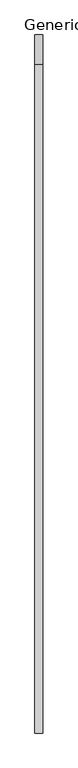
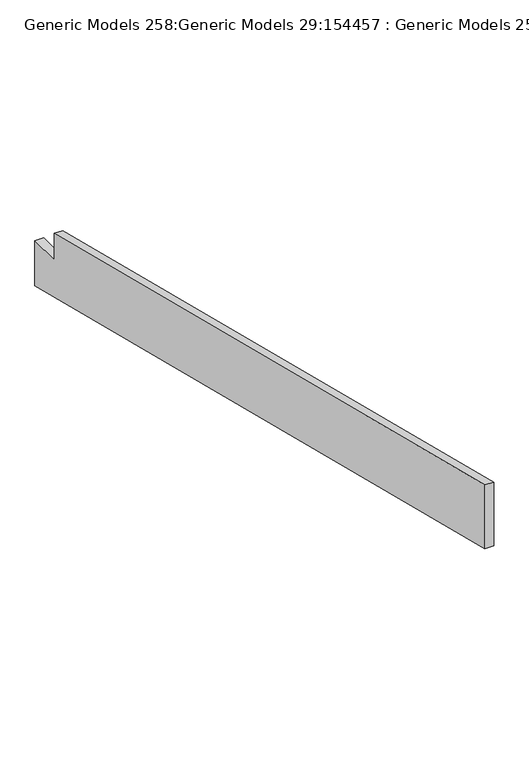
"""IFC4 building model written with IfcOpenShell, lengths in millimetres: proxy geometry, Generic Models 258:Generic Models 29:154457 : Generic Models 258:Generic Models 29:154457."""

from ifc_helpers import new_model, si_unit, frame, origin, place, context, project, spatial, polyline, outline, extrude, source, transform, mapped, element, save


def generic_models_258_generic_models_29_154457_generic_models_30c3a0cf(model_context):
    return source(origin(), model_context, "Body", "SweptSolid", [
        extrude(outline(polyline([(12781.6025207, 4933.3670071), (12781.6025207, 4724.4), (9378.0025207, 5575.3), (9378.0025207, 5869.8443581), (12635.5525207, 5055.4568581), (12635.5525207, 4933.3670071), (12781.6025207, 4933.3670071)])), frame((-2238.496787, 0.0, 0.0), z_axis=(1.0, 0.0, 0.0), x_axis=(0.0, 1.0, 0.0)), (0.0, 0.0, 1.0), 38.1),
    ])


if __name__ == "__main__":
    model = new_model("IFC4")
    model_context = context("Model", 3, world=origin())
    ifc_project = project(units=[si_unit("LENGTHUNIT", "METRE", prefix="MILLI")], contexts=[model_context])
    site = spatial("IfcSite", under=ifc_project)
    building = spatial("IfcBuilding", under=site)
    placement = place(None, origin())
    generic_models_258_generic_models_29_154457_generic_models_shape = generic_models_258_generic_models_29_154457_generic_models_30c3a0cf(model_context)
    element("IfcBuildingElementProxy", 1, Name="Generic Models 258:Generic Models 29:154457 : Generic Models 258:Generic Models 29:154457", ObjectType="Generic Models 258:Generic Models 29:154457 : Generic Models 258:Generic Models 29:154457", at=placement, inside=building, context=model_context, shape_type="MappedRepresentation", body=[
        mapped(generic_models_258_generic_models_29_154457_generic_models_shape, transform((0.0, 0.0, 0.0), x_axis=(1.0, 0.0, 0.0), y_axis=(0.0, 1.0, 0.0), z_axis=(0.0, 0.0, 1.0))),
    ])
    save(model, "model.ifc")

# Revit data of these elements
# Type "Generic Models 258:Generic Models 29:154457 : Generic Models 258:Generic Models 29:154457"
#   NameOverride = "Generic Models 258:Generic Models 29:154457"
#   ObjectTypeOverride = "Generic Models 258:Generic Models 29"
#   Reference = "Generic Models 29"
#   Category = "Generic Models"
#   Tag = "154457"
# Element 1 (IfcBuildingElementProxy, "Generic Models 258:Generic Models 29:154457 : Generic Models 258:Generic Models 29:154457")
#   Materials on its faces: "_STRUCTURAL MEMBER (SEE STRUCT. DWGS) 154"
# Materials
#   "_STRUCTURAL MEMBER (SEE STRUCT. DWGS) 154": class "Unassigned", colour RGB 209 182 141, transparency 0
